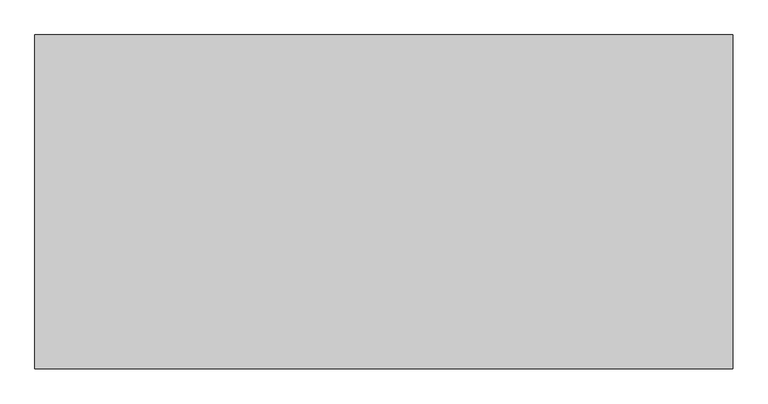
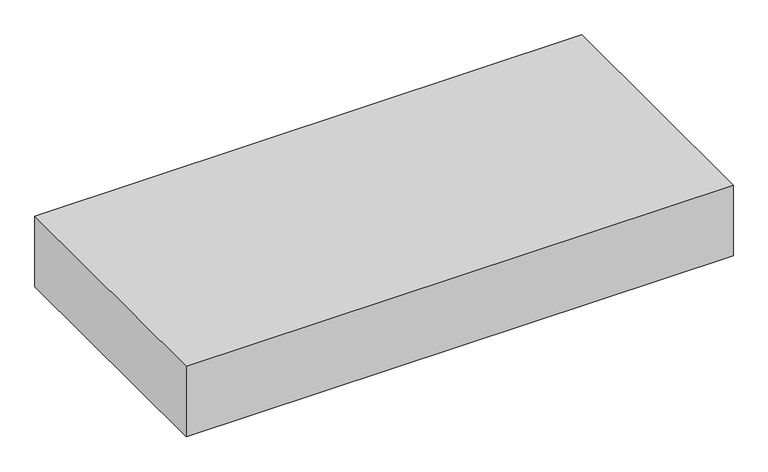
"""IFC4 building model written with IfcOpenShell, lengths in millimetres: proxy geometry, Space Planning Box_hec : Space Planning Box_hec."""

from ifc_helpers import new_model, si_unit, origin, origin_with_axes, place, context, project, spatial, polyline, outline, extrude, source, transform, mapped, element, save


def generic_models_b3b0fa1d(model_context):
    return source(origin(), model_context, "Body", "SweptSolid", [
        extrude(outline(polyline([(21950.0, 10500.0), (21950.0, -10500.0), (-21950.0, -10500.0), (-21950.0, 10500.0), (21950.0, 10500.0)])), origin_with_axes(), (0.0, 0.0, 1.0), 6000.0),
    ])


if __name__ == "__main__":
    model = new_model("IFC4")
    model_context = context("Model", 3, world=origin())
    ifc_project = project(units=[si_unit("LENGTHUNIT", "METRE", prefix="MILLI")], contexts=[model_context])
    site = spatial("IfcSite", under=ifc_project)
    building = spatial("IfcBuilding", under=site)
    placement = place(None, origin())
    generic_models_shape = generic_models_b3b0fa1d(model_context)
    element("IfcBuildingElementProxy", 1, Name="Space Planning Box_hec : Space Planning Box_hec", ObjectType="Space Planning Box_hec : Space Planning Box_hec", at=placement, inside=building, context=model_context, shape_type="MappedRepresentation", body=[
        mapped(generic_models_shape, transform((0.0, 0.0, 0.0), x_axis=(1.0, 0.0, 0.0), y_axis=(0.0, 1.0, 0.0), z_axis=(0.0, 0.0, 1.0))),
    ])
    save(model, "model.ifc")

# Revit data of these elements
# Type "Space Planning Box_hec : Space Planning Box_hec"
#   Type Comments = "..."
#   Room Name [instance default] = "?"
#   Interior Finish [instance default] = ""
#   Exterior Finish [instance default] = ""
#   Department [instance default] = ""
#   Assembly Code = "..."
#   Width [instance default] = 1524 mm
#   Program Area [instance default] = 0 m²
#   Length [instance default] = 1524 mm
#   Height [instance default] = 1524 mm
#   Area [instance default] = 2.32258 m²
#   Fill Color [instance default] = Cyan
#   Default Elevation = 0
# Element 1 (IfcBuildingElementProxy, "Space Planning Box_hec : Space Planning Box_hec")
#   Room Name = "Corridor"
#   Interior Finish = "IF2-1"
#   Exterior Finish = "EF1"
#   Department = "AR"
#   Width = 43900 mm
#   Length = 21000 mm
#   Height = 6000 mm
#   Area = 921.9 m²
#   Fill Color = Lavender
#   Materials on its faces: "Lavender"
# Materials
#   "Cyan": class "Generic", colour RGB 0 255 255, transparency 0.2, Cost = 0
#   "Lavender": class "Generic", colour RGB 186 85 211, transparency 0.2, Cost = 0
